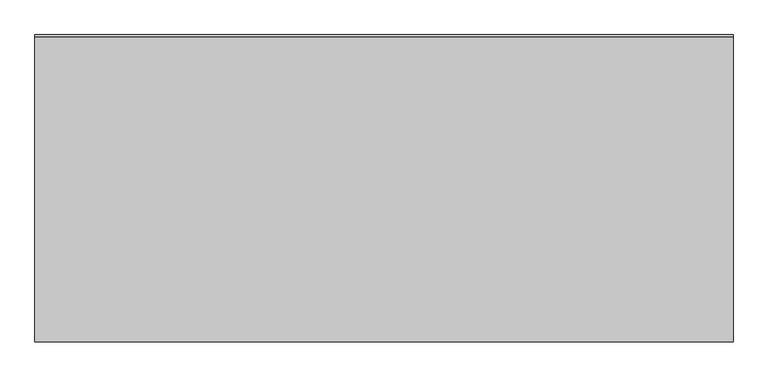
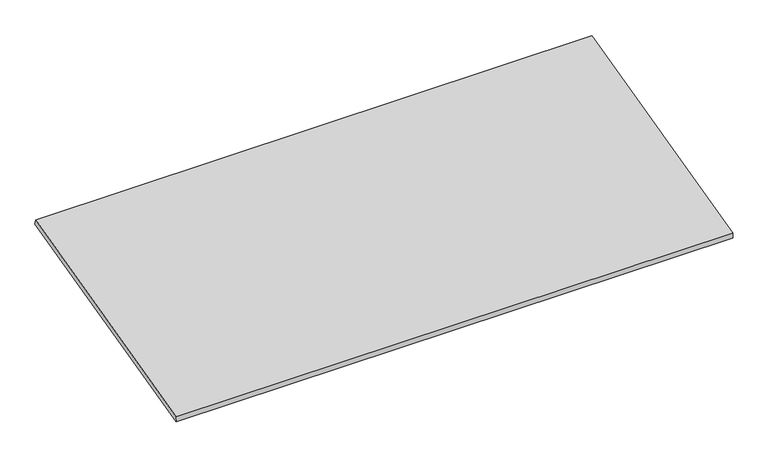
"""IFC4 building model written with IfcOpenShell, lengths in millimetres: proxy geometry, Gypsum012 968 : Gypsum012 968."""

from ifc_helpers import new_model, si_unit, frame, origin, place, context, project, spatial, polyline, outline, extrude, source, transform, mapped, element, save


def generic_models_edbfed62(model_context):
    return source(origin(), model_context, "Body", "SweptSolid", [
        extrude(outline(polyline([(8858.3726979, 42998.7226562), (8857.883325, 43018.0404079), (9733.2922309, 43237.0426118), (9737.9368073, 43218.4770293), (8858.3726979, 42998.7226562)])), frame((3694.2883192, 0.0, 0.0), z_axis=(1.0, 0.0, 0.0), x_axis=(0.0, 1.0, 0.0)), (0.0, 0.0, 1.0), 2000.0),
    ])


if __name__ == "__main__":
    model = new_model("IFC4")
    model_context = context("Model", 3, world=origin())
    ifc_project = project(units=[si_unit("LENGTHUNIT", "METRE", prefix="MILLI")], contexts=[model_context])
    site = spatial("IfcSite", under=ifc_project)
    building = spatial("IfcBuilding", under=site)
    placement = place(None, origin())
    generic_models_shape = generic_models_edbfed62(model_context)
    element("IfcBuildingElementProxy", 1, Name="Gypsum012 968 : Gypsum012 968", ObjectType="Gypsum012 968 : Gypsum012 968", at=placement, inside=building, context=model_context, shape_type="MappedRepresentation", body=[
        mapped(generic_models_shape, transform((0.0, 0.0, 0.0), x_axis=(1.0, 0.0, 0.0), y_axis=(0.0, 1.0, 0.0), z_axis=(0.0, 0.0, 1.0))),
    ])
    save(model, "model.ifc")

# Revit data of these elements
# Type "Gypsum012 968 : Gypsum012 968"
#   NameOverride = "Gypsum012"
# Element 1 (IfcBuildingElementProxy, "Gypsum012 968 : Gypsum012 968")
#   Materials on its faces: "5/8\"  GYPSUM BOARD"
# Materials
#   "5/8\"  GYPSUM BOARD": class "Unassigned", colour RGB 255 255 255, transparency 0, Cost = 0
